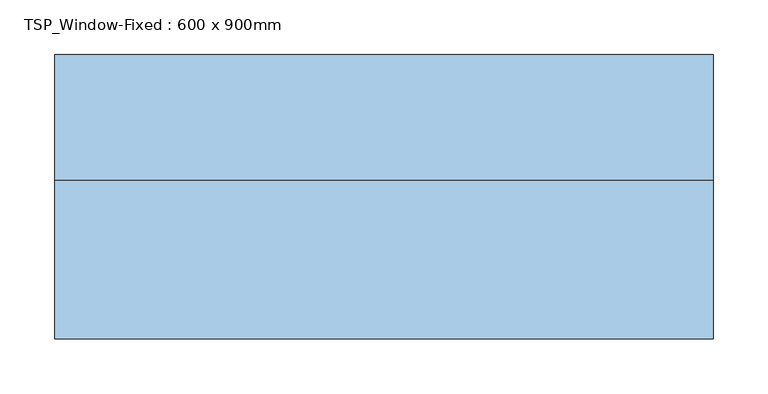
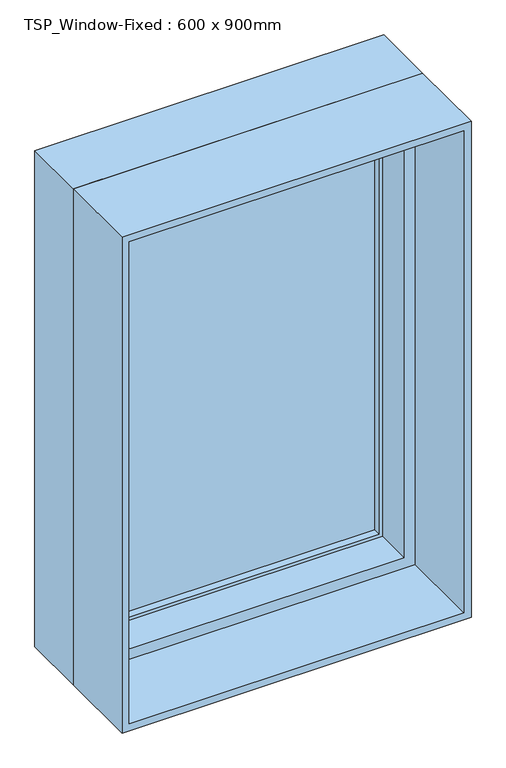
"""IFC4 building model written with IfcOpenShell, lengths in millimetres: window geometry, TSP_Window-Fixed : 600 x 900mm."""

from ifc_helpers import new_model, si_unit, frame, origin, place, context, project, spatial, polyline, outline, extrude, faceted_brep, source, transform, mapped, element, save


def tsp_window_fixed_600_x_900mm_725ff1cf(model_context):
    return source(origin(), model_context, "Body", "SolidModel", [
        faceted_brep([(300.0, 24.75, 1800.0), (300.0, 139.05, 1800.0), (-300.0, 139.05, 1800.0), (-300.0, 24.75, 1800.0), (-300.0, 139.05, 900.0), (-300.0, 24.75, 900.0), (300.0, 139.05, 900.0), (300.0, 24.75, 900.0), (268.25, 24.75, 1768.25), (268.25, 24.75, 931.75), (-268.25, 24.75, 931.75), (-268.25, 24.75, 1768.25), (-287.3, 139.05, 1787.3), (-287.3, 139.05, 912.7), (287.3, 139.05, 912.7), (287.3, 139.05, 1787.3), (268.25, 88.25, 1768.25), (-268.25, 88.25, 1768.25), (287.3, 88.25, 1787.3), (-287.3, 88.25, 1787.3), (-268.25, 88.25, 931.75), (-287.3, 88.25, 912.7), (268.25, 88.25, 931.75), (287.3, 88.25, 912.7)], [[[0, 1, 2, 3]], [[3, 2, 4, 5]], [[5, 4, 6, 7]], [[3, 5, 7, 0], [8, 9, 10, 11]], [[7, 6, 1, 0]], [[1, 6, 4, 2], [12, 13, 14, 15]], [[16, 8, 11, 17]], [[15, 18, 19, 12]], [[17, 11, 10, 20]], [[12, 19, 21, 13]], [[20, 10, 9, 22]], [[13, 21, 23, 14]], [[22, 9, 8, 16]], [[18, 23, 21, 19], [17, 20, 22, 16]], [[14, 23, 18, 15]]]),
        extrude(outline(polyline([(1800.0, -300.0), (900.0, -300.0), (900.0, 300.0), (1800.0, 300.0), (1800.0, -300.0)]), holes=[polyline([(1787.3, 287.3), (912.7, 287.3), (912.7, -287.3), (1787.3, -287.3), (1787.3, 287.3)])]), frame((0.0, -120.0, 0.0), z_axis=(0.0, 1.0, 0.0), x_axis=(0.0, 0.0, 1.0)), (0.0, 0.0, 1.0), 144.75),
        extrude(outline(polyline([(912.7, 287.3), (1787.3, 287.3), (1787.3, -287.3), (912.7, -287.3), (912.7, 287.3)]), holes=[polyline([(938.1, -261.9), (1761.9, -261.9), (1761.9, 261.9), (938.1, 261.9), (938.1, -261.9)])]), frame((0.0, 88.25, 0.0), z_axis=(0.0, 1.0, 0.0), x_axis=(0.0, 0.0, 1.0)), (0.0, 0.0, 1.0), 44.45),
        extrude(outline(polyline([(261.9, 120.0), (261.9, 113.65), (-261.9, 113.65), (-261.9, 120.0), (261.9, 120.0)])), frame((0.0, 0.0, 938.1), z_axis=(0.0, 0.0, 1.0), x_axis=(1.0, 0.0, 0.0)), (0.0, 0.0, 1.0), 823.8),
        extrude(outline(polyline([(-261.9, 100.95), (-261.9, 107.3), (261.9, 107.3), (261.9, 100.95), (-261.9, 100.95)])), frame((0.0, 0.0, 938.1), z_axis=(0.0, 0.0, 1.0), x_axis=(1.0, 0.0, 0.0)), (0.0, 0.0, 1.0), 823.8),
    ])


if __name__ == "__main__":
    model = new_model("IFC4")
    model_context = context("Model", 3, world=origin())
    ifc_project = project(units=[si_unit("LENGTHUNIT", "METRE", prefix="MILLI")], contexts=[model_context])
    site = spatial("IfcSite", under=ifc_project)
    building = spatial("IfcBuilding", under=site)
    placement = place(None, origin())
    tsp_window_fixed_600_x_900mm_shape = tsp_window_fixed_600_x_900mm_725ff1cf(model_context)
    element("IfcWindow", 1, ObjectType="TSP_Window-Fixed : 600 x 900mm", at=placement, inside=building, context=model_context, shape_type="MappedRepresentation", body=[
        mapped(tsp_window_fixed_600_x_900mm_shape, transform((0.0, 0.0, 0.0), x_axis=(1.0, 0.0, 0.0), y_axis=(0.0, 1.0, 0.0), z_axis=(0.0, 0.0, 1.0))),
    ])
    save(model, "model.ifc")

# Revit data of these elements
# Type "TSP_Window-Fixed : 600 x 900mm"
#   Type Mark = "HS 2412 F134"
#   Fire Rating = "0.5h"
#   Assembly Code = "B2020100"
#   Analytic Construction = "Double glazing - domestic"
#   Window Inset [instance default] = 0 mm
#   Wall Thickness [instance default] = 150 mm
#   Visual Light Transmittance = 0.81
#   Thermal Resistance (R) = 0.319569 (m²·K)/W
#   Solar Heat Gain Coefficient = 0.76
#   Rough Width = 615 mm
#   Rough Height = 915 mm
#   Interior Wall Closure [instance default] = 54.75 mm
#   Height = 900 mm
#   Heat Transfer Coefficient (U) = 3.12929 W/(m²·K)
#   Frame Extension [instance default] = 6.35 mm
#   Exterior Wall Closure [instance default] = 31.75 mm
#   Extension Jamb [instance default] = 54.75 mm
#   Default Sill Height = 900 mm
#   Width = 600 mm
#   Muntin Visibility = yes
#   Interior Trim Visibility [instance default] = yes
#   Exterior Trim Visibility [instance default] = yes
#   Extension Jamb Visibility [instance default] = yes
#   Interior Trim Material = Wood - Stained
#   Interior Frame Material = Wood - Stained
#   Glass Panel Material = Glass
#   Exterior Trim Material = Clad - White
#   Exterior Frame Material = Clad - White
#   Wall Closure = (empty or 0)
# Element 1 (IfcWindow, "TSP_Window-Fixed : 600 x 900mm")
#   Wall Thickness = 240 mm
#   Extension Jamb = 144.75 mm
#   Materials on its faces: "Wood - Stained", "Glass", "Clad - White"
# Materials
#   "Wood - Stained": class "Wood", colour RGB 224 178 126, transparency 0, Cost = 0
#   "Glass": class "Glass", colour RGB 0 128 192, transparency 0.9, Description = "Soda Lime Glass", Cost = 0
#   "Clad - White": class "Wood", colour RGB 242 242 238, transparency 0, Cost = 0
